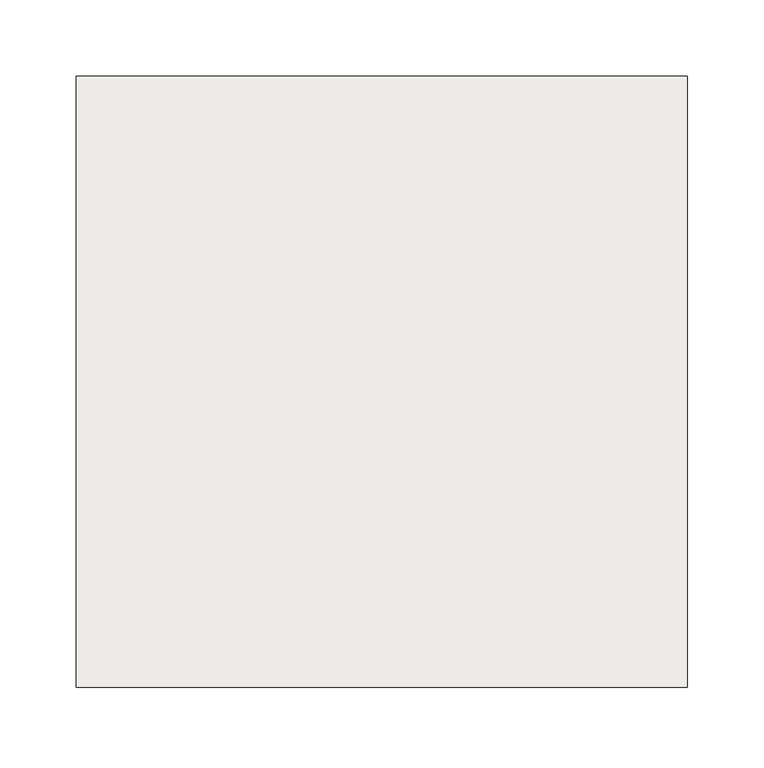
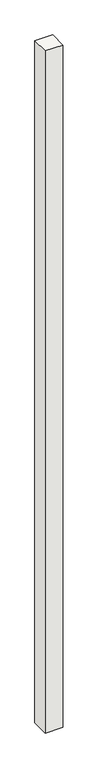
"""IFC4 building model written with IfcOpenShell, lengths in millimetres: slab geometry, NLRS_17_SFO_TLB_funderingspaal geheid beton prefab-AV-MMBPC_gen_rsf : heipaal beton prefab_gen__bxh 400x400."""

from ifc_helpers import new_model, si_unit, frame, origin, place, context, project, spatial, polyline, outline, extrude, source, transform, mapped, element, save


def slab_98706cf3(model_context):
    return source(origin(), model_context, "Body", "SweptSolid", [
        extrude(outline(polyline([(200.0, -200.0), (-200.0, -200.0), (-200.0, 200.0), (200.0, 200.0), (200.0, -200.0)])), frame((0.0, 0.0, -20000.0), z_axis=(0.0, 0.0, 1.0), x_axis=(1.0, 0.0, 0.0)), (0.0, 0.0, 1.0), 16280.0),
    ])


if __name__ == "__main__":
    model = new_model("IFC4")
    model_context = context("Model", 3, world=origin())
    ifc_project = project(units=[si_unit("LENGTHUNIT", "METRE", prefix="MILLI")], contexts=[model_context])
    site = spatial("IfcSite", under=ifc_project)
    building = spatial("IfcBuilding", under=site)
    placement = place(None, origin())
    slab_shape = slab_98706cf3(model_context)
    element("IfcSlab", 1, ObjectType="NLRS_17_SFO_TLB_funderingspaal geheid beton prefab-AV-MMBPC_gen_rsf : heipaal beton prefab_gen__bxh 400x400", at=placement, inside=building, context=model_context, shape_type="MappedRepresentation", body=[
        mapped(slab_shape, transform((0.0, 0.0, 0.0), x_axis=(1.0, 0.0, 0.0), y_axis=(0.0, 1.0, 0.0), z_axis=(0.0, 0.0, 1.0))),
    ])
    save(model, "model.ifc")

# Revit data of these elements
# Type "NLRS_17_SFO_TLB_funderingspaal geheid beton prefab-AV-MMBPC_gen_rsf : heipaal beton prefab_gen__bxh 400x400"
#   Export Type to IFC As = "IfcPile"
#   Type IfcGUID = "10$Kfo5uPCAOPJEOo5LE_W"
#   Type Comments = "prefab heipaal 400x400"
#   Model = " "
#   Manufacturer = " "
#   Description = "prefab heipaal 400x400"
#   Assembly Code = "17.21"
#   Width = 400 mm
#   Slanted Angle [instance default] = 0.00°
#   NLRS_S_draagvermogen_trek [instance default] = 0.00 kN
#   NLRS_S_draagvermogen_druk [instance default] = 0.00 kN
#   NLRS_C_lengte [instance default] = 1660 mm
#   NLRS_C_hoogte = 400 mm
#   NLRS_C_breedte = 400 mm
#   Height [instance default] = 1660 mm
#   Length [instance default] = 1660 mm
#   Angle [instance default] = 0.00°
#   Slanted [instance default] = 0
#   Structural Material = NLRS_f2_beton prefab_gen_rsf
#   Keynote = ""
# Element 1 (IfcSlab, "NLRS_17_SFO_TLB_funderingspaal geheid beton prefab-AV-MMBPC_gen_rsf : heipaal beton prefab_gen__bxh 400x400")
#   NLRS_C_lengte = 16280 mm
#   Height = 16280 mm
#   Length = 16280 mm
#   Materials on its faces: "NLRS_f2_beton prefab_gen_rsf"
# Materials
#   "NLRS_f2_beton prefab_gen_rsf": class "F - Niet gebakken kunststeen", colour RGB 129 133 118, transparency 0, Keynote = "f2", Manufacturer = "Revit Standards Foundation", URL = "www.revitstandards.org", Description = "beton prefab", Cost = 0
